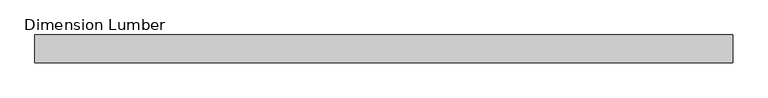
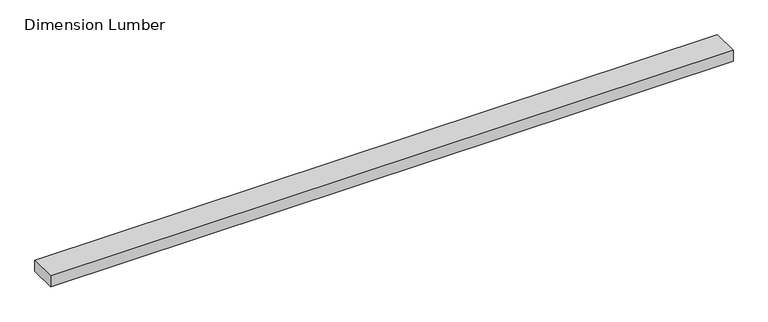
"""IFC4 building model written with IfcOpenShell, lengths in millimetres: beam geometry, Dimension Lumber : Top Supporting Lumbers."""

from ifc_helpers import new_model, si_unit, frame, origin, place, context, project, spatial, polyline, outline, extrude, source, transform, mapped, element, save


def dimension_lumber_901b61d8(model_context):
    return source(origin(), model_context, "Body", "SweptSolid", [
        extrude(outline(polyline([(1117.6, 44.45), (1117.6, -44.45), (-1117.6, -44.45), (-1117.6, 44.45), (1117.6, 44.45)])), frame((0.0, 0.0, -19.05), z_axis=(0.0, 0.0, 1.0), x_axis=(1.0, 0.0, 0.0)), (0.0, 0.0, 1.0), 38.1),
    ])


if __name__ == "__main__":
    model = new_model("IFC4")
    model_context = context("Model", 3, world=origin())
    ifc_project = project(units=[si_unit("LENGTHUNIT", "METRE", prefix="MILLI")], contexts=[model_context])
    site = spatial("IfcSite", under=ifc_project)
    building = spatial("IfcBuilding", under=site)
    placement = place(None, origin())
    dimension_lumber_shape = dimension_lumber_901b61d8(model_context)
    element("IfcBeam", 1, ObjectType="Dimension Lumber : Top Supporting Lumbers", at=placement, inside=building, context=model_context, shape_type="MappedRepresentation", body=[
        mapped(dimension_lumber_shape, transform((0.0, 0.0, 0.0), x_axis=(1.0, 0.0, 0.0), y_axis=(0.0, 1.0, 0.0), z_axis=(0.0, 0.0, 1.0))),
    ])
    save(model, "model.ifc")

# Revit data of these elements
# Type "Dimension Lumber : Top Supporting Lumbers"
#   Assembly Code = "B10"
#   A = 0.0364583 SF
#   Length [instance default] = 5' - 0"
#   b = 0' - 3 1/2"
#   d = 0' - 1 1/2"
#   Structural Material [instance default] = Softwood, Lumber
# Element 1 (IfcBeam, "Dimension Lumber : Top Supporting Lumbers")
#   Structural Material = Douglas Fir #2
#   Materials on its faces: "Douglas Fir #2"
# Materials
#   "Softwood, Lumber": class "Wood", colour RGB 223 192 134, transparency 0, Description = "Pinus Echinata", Cost = 0
#   "Douglas Fir #2": class "Wood", colour RGB 223 192 134, transparency 0, Description = "Pinus Echinata", Cost = 0
